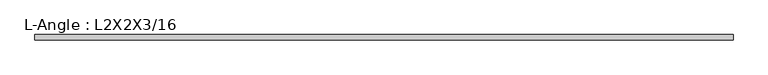
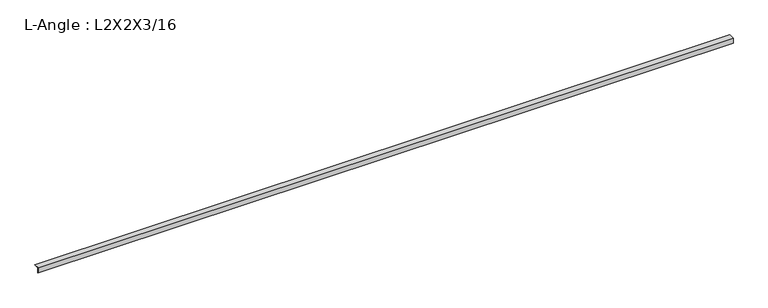
"""IFC4 building model written with IfcOpenShell, lengths in millimetres: beam geometry, L-Angle : L2X2X3/16."""

import ifcopenshell
import ifcopenshell.guid

model = None  # the IFC model being written
_history = None  # IfcOwnerHistory: only IFC2X3 demands one
_inside = {}  # id of a spatial element -> (the spatial element, [elements in it])
_under = {}  # id of a project, library or spatial element -> (it, [spatial elements below it])
_declared = {}  # id of a project -> (the project, [libraries it declares])
_typed = {}  # id of a type object -> (the type object, [elements of that type])
_made_of = {}  # id of a material, layer set ... -> (it, [elements and type objects made of it])


def new_model(schema):
    """Start an empty IFC model of exactly this schema.

    Asked for "IFC4X3", IfcOpenShell would pick the latest addendum, in which some entities
    have other attributes; the version numbers below select the first issue.
    IFC2X3 requires an IfcOwnerHistory on every rooted entity: one is made here for all.
    """
    global model, _history
    if schema == "IFC4X3":
        model = ifcopenshell.file(schema_version=(4, 3, 0, 0))
    else:
        model = ifcopenshell.file(schema=schema)
    _inside.clear()
    _under.clear()
    _declared.clear()
    _typed.clear()
    _made_of.clear()
    _history = None
    if model.schema == "IFC2X3":
        org = make("IfcOrganization", Name="unknown")
        user = make(
            "IfcPersonAndOrganization",
            ThePerson=make("IfcPerson", FamilyName="unknown"),
            TheOrganization=org,
        )
        app = make(
            "IfcApplication",
            ApplicationDeveloper=org,
            Version="unknown",
            ApplicationFullName="unknown",
            ApplicationIdentifier="unknown",
        )
        _history = make(
            "IfcOwnerHistory",
            OwningUser=user,
            OwningApplication=app,
            ChangeAction="ADDED",
            CreationDate=0,
        )
    return model


def make(cls, **values):
    """One entity of the class cls with the attributes given. An attribute that is None is left unset."""
    return model.create_entity(
        cls, **{name: value for name, value in values.items() if value is not None}
    )


def rooted(cls, **values):
    """An entity with a GlobalId (a new one), such as an element, a storey or a relation."""
    return make(cls, GlobalId=ifcopenshell.guid.new(), OwnerHistory=_history, **values)


def si_unit(unit_type, name, prefix=None):
    """IfcSIUnit, for example si_unit("LENGTHUNIT", "METRE", prefix="MILLI")."""
    return make("IfcSIUnit", UnitType=unit_type, Prefix=prefix, Name=name)


def assignment(units):
    """IfcUnitAssignment: the units of a project."""
    return None if units is None else make("IfcUnitAssignment", Units=units)


def point(xyz):
    """IfcCartesianPoint."""
    return None if xyz is None else make("IfcCartesianPoint", Coordinates=xyz)


def direction(xyz):
    """IfcDirection."""
    return None if xyz is None else make("IfcDirection", DirectionRatios=xyz)


def frame(location, z_axis=None, x_axis=None):
    """IfcAxis2Placement3D, a coordinate frame: its origin and axes. An axis left out is left unset."""
    return make(
        "IfcAxis2Placement3D",
        Location=point(location),
        Axis=direction(z_axis),
        RefDirection=direction(x_axis),
    )


def frame_2d(location, x_axis=None):
    """IfcAxis2Placement2D, a coordinate frame in the plane: its origin and x axis."""
    return make(
        "IfcAxis2Placement2D", Location=point(location), RefDirection=direction(x_axis)
    )


def origin():
    """The frame at (0, 0, 0) with its axes left unset."""
    return frame((0.0, 0.0, 0.0))


def place(relative_to, where):
    """IfcLocalPlacement: puts the frame where relative to a parent placement (None: the world)."""
    return make(
        "IfcLocalPlacement", PlacementRelTo=relative_to, RelativePlacement=where
    )


def context(
    kind, dimensions, precision=None, world=None, true_north=None, identifier=None
):
    """IfcGeometricRepresentationContext, for example the 3D "Model" context."""
    return make(
        "IfcGeometricRepresentationContext",
        ContextIdentifier=identifier,
        ContextType=kind,
        CoordinateSpaceDimension=dimensions,
        Precision=precision,
        WorldCoordinateSystem=world,
        TrueNorth=true_north,
    )


def project(units=None, contexts=None):
    """IfcProject with its units and contexts."""
    return rooted(
        "IfcProject",
        Name="project",
        RepresentationContexts=contexts,
        UnitsInContext=assignment(units),
    )


def spatial(cls, under=None, at=None, **own):
    """A site, building, storey or space (cls), placed at a placement, below another one or the project."""
    s = rooted(cls, ObjectPlacement=at, **own)
    if under is not None:
        _under.setdefault(under.id(), (under, []))[1].append(s)
    return s


def polyline(points):
    """IfcPolyline through the points."""
    return make("IfcPolyline", Points=[point(p) for p in points])


def circle_curve(where, radius):
    """IfcCircle in the frame where."""
    return make("IfcCircle", Position=where, Radius=radius)


def trimmed(basis, trim1, trim2, sense, master):
    """IfcTrimmedCurve: the piece of a basis curve between two trims."""
    return make(
        "IfcTrimmedCurve",
        BasisCurve=basis,
        Trim1=trim1,
        Trim2=trim2,
        SenseAgreement=sense,
        MasterRepresentation=master,
    )


def segment(curve, same_sense, transition):
    """IfcCompositeCurveSegment."""
    return make(
        "IfcCompositeCurveSegment",
        Transition=transition,
        SameSense=same_sense,
        ParentCurve=curve,
    )


def composite_curve(segments, self_intersect=None):
    """IfcCompositeCurve: segments joined end to end."""
    return make("IfcCompositeCurve", Segments=segments, SelfIntersect=self_intersect)


def outline(outer, holes=None, kind="AREA"):
    """IfcArbitraryClosedProfileDef: a profile drawn as a closed curve; with holes, ...WithVoids."""
    if holes is None:
        return make("IfcArbitraryClosedProfileDef", ProfileType=kind, OuterCurve=outer)
    return make(
        "IfcArbitraryProfileDefWithVoids",
        ProfileType=kind,
        OuterCurve=outer,
        InnerCurves=holes,
    )


def extrude(swept, where, along, depth):
    """IfcExtrudedAreaSolid: the profile swept, set in the frame where, extruded along a direction by depth."""
    return make(
        "IfcExtrudedAreaSolid",
        SweptArea=swept,
        Position=where,
        ExtrudedDirection=direction(along),
        Depth=depth,
    )


def shape(context_of_items, identifier, shape_type, items):
    """IfcShapeRepresentation: the items that make up one representation, for example the "Body"."""
    return make(
        "IfcShapeRepresentation",
        ContextOfItems=context_of_items,
        RepresentationIdentifier=identifier,
        RepresentationType=shape_type,
        Items=items,
    )


def source(mapping_origin, context_of_items, identifier, shape_type, items):
    """IfcRepresentationMap: a shape defined once, which mapped items show again and again."""
    return make(
        "IfcRepresentationMap",
        MappingOrigin=mapping_origin,
        MappedRepresentation=shape(context_of_items, identifier, shape_type, items),
    )


def transform(
    local_origin,
    x_axis=None,
    y_axis=None,
    z_axis=None,
    scale=None,
    scale2=None,
    scale3=None,
    uniform=True,
):
    """IfcCartesianTransformationOperator3D, or its non-uniform kind. x_axis, y_axis, z_axis: its Axis1, 2, 3."""
    if uniform:
        return make(
            "IfcCartesianTransformationOperator3D",
            Axis1=direction(x_axis),
            Axis2=direction(y_axis),
            LocalOrigin=point(local_origin),
            Scale=scale,
            Axis3=direction(z_axis),
        )
    return make(
        "IfcCartesianTransformationOperator3DnonUniform",
        Axis1=direction(x_axis),
        Axis2=direction(y_axis),
        LocalOrigin=point(local_origin),
        Scale=scale,
        Axis3=direction(z_axis),
        Scale2=scale2,
        Scale3=scale3,
    )


def mapped(mapping_source, mapping_target):
    """IfcMappedItem: shows the shape of a source again, moved by a transform."""
    return make(
        "IfcMappedItem", MappingSource=mapping_source, MappingTarget=mapping_target
    )


def made_of(thing, what):
    """Note that an element or type object is made of a material, layer set ...; save() writes the relation."""
    if what is not None:
        _made_of.setdefault(what.id(), (what, []))[1].append(thing)
    return thing


def element(
    cls,
    number,
    at=None,
    inside=None,
    cuts=None,
    type_object=None,
    material=None,
    context=None,
    identifier="Body",
    shape_type=None,
    held_by="IfcProductDefinitionShape",
    body=None,
    shapes=None,
    **own,
):
    """One element of the class cls, such as IfcWall. Its Tag is "e" and its number.

    at: its placement. inside: the storey or other place that contains it. cuts: it is an
    opening in that element (IfcRelVoidsElement). A single representation is given by context,
    identifier, shape_type and body (its items); several are given by shapes. held_by: the class
    of the entity that holds the representations. save() writes the other relations.
    """
    e = rooted(cls, Tag="e%d" % number, ObjectPlacement=at, **own)
    if body is not None:
        shapes = [shape(context, identifier, shape_type, body)]
    if shapes is not None:
        e.Representation = make(held_by, Representations=shapes)
    if inside is not None:
        _inside.setdefault(inside.id(), (inside, []))[1].append(e)
    if cuts is not None:
        rooted(
            "IfcRelVoidsElement", RelatingBuildingElement=cuts, RelatedOpeningElement=e
        )
    if type_object is not None:
        _typed.setdefault(type_object.id(), (type_object, []))[1].append(e)
    return made_of(e, material)


def aggregate(whole, parts):
    """IfcRelAggregates: a whole, such as a stair, and the parts it consists of."""
    return rooted("IfcRelAggregates", RelatingObject=whole, RelatedObjects=parts)


def save(model, path):
    """Write the relations noted so far, then the file.

    IfcRelAggregates (storeys below a building ...), IfcRelContainedInSpatialStructure (elements
    in a storey), IfcRelDefinesByType, IfcRelAssociatesMaterial and IfcRelDeclares: one each for
    every whole, place, type object, material and project.
    """
    for whole, parts in _under.values():
        aggregate(whole, parts)
    for where, things in _inside.values():
        rooted(
            "IfcRelContainedInSpatialStructure",
            RelatedElements=things,
            RelatingStructure=where,
        )
    for kind, things in _typed.values():
        rooted("IfcRelDefinesByType", RelatedObjects=things, RelatingType=kind)
    for what, things in _made_of.values():
        rooted("IfcRelAssociatesMaterial", RelatedObjects=things, RelatingMaterial=what)
    for by, libraries in _declared.values():
        rooted("IfcRelDeclares", RelatingContext=by, RelatedDefinitions=libraries)
    model.write(path)


def l_angle_l2x2x3_16_c91ffc3e(model_context):
    return source(origin(), model_context, "Body", "SweptSolid", [
        extrude(outline(composite_curve([segment(polyline([(-14.2494, 14.2494), (36.5506, 14.2494)]), True, "CONTINUOUS"), segment(trimmed(circle_curve(frame_2d((31.7881, 14.2494)), 4.7625), [point((36.5506, 14.2494))], [point((31.7881, 9.4869))], False, "CARTESIAN"), True, "CONTINUOUS"), segment(polyline([(31.7881, 9.4869), (-4.7244, 9.4869)]), True, "CONTINUOUS"), segment(trimmed(circle_curve(frame_2d((-4.7244, 4.7244)), 4.7625), [point((-4.7244, 9.4869))], [point((-9.4869, 4.7244))], True, "CARTESIAN"), True, "CONTINUOUS"), segment(polyline([(-9.4869, 4.7244), (-9.4869, -31.7881)]), True, "CONTINUOUS"), segment(trimmed(circle_curve(frame_2d((-14.2494, -31.7881)), 4.7625), [point((-9.4869, -31.7881))], [point((-14.2494, -36.5506))], False, "CARTESIAN"), True, "CONTINUOUS"), segment(polyline([(-14.2494, -36.5506), (-14.2494, 14.2494)]), True, "CONTINUOUS")], self_intersect=False)), frame((-3265.4875, 0.0, 0.0), z_axis=(1.0, 0.0, 0.0), x_axis=(0.0, 1.0, 0.0)), (0.0, 0.0, 1.0), 6359.525),
    ])


if __name__ == "__main__":
    model = new_model("IFC4")
    model_context = context("Model", 3, world=origin())
    ifc_project = project(units=[si_unit("LENGTHUNIT", "METRE", prefix="MILLI")], contexts=[model_context])
    site = spatial("IfcSite", under=ifc_project)
    building = spatial("IfcBuilding", under=site)
    placement = place(None, origin())
    l_angle_l2x2x3_16_shape = l_angle_l2x2x3_16_c91ffc3e(model_context)
    element("IfcBeam", 1, ObjectType="L-Angle : L2X2X3/16", at=placement, inside=building, context=model_context, shape_type="MappedRepresentation", body=[
        mapped(l_angle_l2x2x3_16_shape, transform((0.0, 0.0, 0.0), x_axis=(1.0, 0.0, 0.0), y_axis=(0.0, 1.0, 0.0), z_axis=(0.0, 0.0, 1.0))),
    ])
    save(model, "model.ifc")

# Revit data of these elements
# Type "L-Angle : L2X2X3/16"
#   Assembly Code = "B10"
#   k = 0' - 0 7/16"
#   W = 2.44
#   Start Extension Calculation [instance default] = 10' - 0"
#   Start Extension [instance default] = -0' - 0 1/2"
#   End Extension Calculation [instance default] = 10' - 0"
#   End Extension [instance default] = -0' - 0 1/2"
#   Length [instance default] = 5' - 0"
#   b = 0' - 2"
#   d = 0' - 2"
#   t = 0' - 0 3/16"
#   x = 0' - 0.561"
#   y = 0' - 0.561"
#   A = 0.00496528 SF
#   Structural Material [instance default] = Metal - Steel - ASTM A36
# Element 1 (IfcBeam, "L-Angle : L2X2X3/16")
#   Structural Material = STRUCTURAL STEEL - SEE STRUCT. DWGS
#   Materials on its faces: "STRUCTURAL STEEL - SEE STRUCT. DWGS"
# Materials
#   "Metal - Steel - ASTM A36": class "Metal", colour RGB 199 199 199, transparency 0
#   "STRUCTURAL STEEL - SEE STRUCT. DWGS": class "Metal", colour RGB 137 146 153, transparency 0, Description = "Steel, mill finish", Cost = 0
